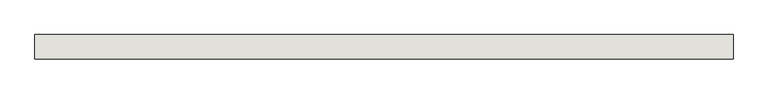
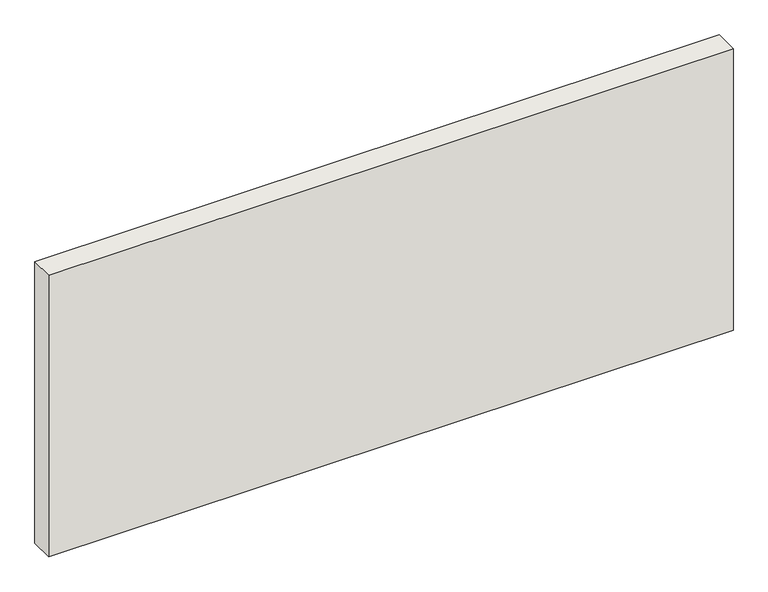
"""IFC4 building model written with IfcOpenShell, lengths in millimetres: wall geometry, Holzwand."""

from ifc_helpers import new_model, si_unit, origin, origin_with_axes, place, context, project, spatial, polyline, outline, extrude, source, transform, mapped, element, save


def wall_f1536983(model_context):
    return source(origin(), model_context, "Body", "SweptSolid", [
        extrude(outline(polyline([(5750.0, 200.0), (5750.0, 0.0), (0.0, 0.0), (0.0, 200.0), (5750.0, 200.0)])), origin_with_axes(), (0.0, 0.0, 1.0), 2500.0),
    ])


if __name__ == "__main__":
    model = new_model("IFC4")
    model_context = context("Model", 3, world=origin())
    ifc_project = project(units=[si_unit("LENGTHUNIT", "METRE", prefix="MILLI")], contexts=[model_context])
    site = spatial("IfcSite", under=ifc_project)
    building = spatial("IfcBuilding", under=site)
    placement = place(None, origin())
    wall_shape = wall_f1536983(model_context)
    element("IfcWall", 1, ObjectType="Holzwand", at=placement, inside=building, context=model_context, shape_type="MappedRepresentation", body=[
        mapped(wall_shape, transform((0.0, 0.0, 0.0), x_axis=(1.0, 0.0, 0.0), y_axis=(0.0, 1.0, 0.0), z_axis=(0.0, 0.0, 1.0))),
    ])
    save(model, "model.ifc")

# Revit data of these elements
# Element 1 (IfcWall, "Holzwand")
#   Materials on its faces: "holzschalung"
# Materials
#   "holzschalung": class "Unassigned", colour RGB 128 128 128, transparency 0
